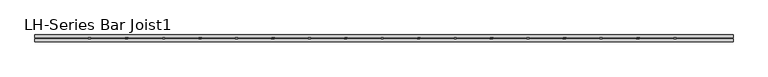
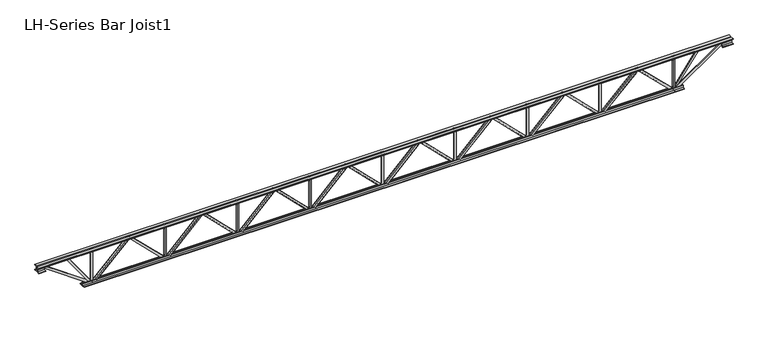
"""IFC4 building model written with IfcOpenShell, lengths in millimetres: beam geometry, LH-Series Bar Joist1 : 32LH-SP8."""

from ifc_helpers import new_model, si_unit, frame, origin, place, context, project, spatial, polyline, outline, extrude, faceted_brep, source, transform, mapped, element, save


def lh_series_bar_joist1_18190fb8(model_context):
    return source(origin(), model_context, "Body", "SolidModel", [
        extrude(outline(polyline([(406.4, 3276.6), (406.4, 3225.8), (323.85, 3225.8), (312.7375, 3236.9125), (-312.7375, 3236.9125), (-323.85, 3225.8), (-406.4, 3225.8), (-406.4, 3276.6), (406.4, 3276.6)])), frame((0.0, -12.7, 0.0), z_axis=(0.0, 1.0, 0.0), x_axis=(0.0, 0.0, 1.0)), (0.0, 0.0, 1.0), 25.4),
        faceted_brep([(3251.2, 0.0, -355.6), (3251.2, 0.0, -406.4), (3251.2, 12.7, -406.4), (3251.2, 12.7, -355.6), (3236.3210245, 0.0, -355.6), (2474.3210245, 0.0, 406.4), (2413.0, 0.0, 406.4), (2413.0, 0.0, 355.6), (2453.2789755, 0.0, 355.6), (3215.2789755, 0.0, -406.4), (3215.2789755, 12.7, -406.4), (3151.7789755, 12.7, -342.9), (3160.7592316, 12.7, -333.9197439), (2474.9592316, 12.7, 351.8802561), (2465.9789755, 12.7, 342.9), (2453.2789755, 12.7, 355.6), (2413.0, 12.7, 355.6), (2413.0, 12.7, 406.4), (2474.3210245, 12.7, 406.4), (3236.3210245, 12.7, -355.6), (2465.9789755, 50.8, 342.9), (3151.7789755, 50.8, -342.9), (3160.7592316, 50.8, -333.9197439), (2474.9592316, 50.8, 351.8802561)], [[[0, 1, 2, 3]], [[1, 0, 4, 5, 6, 7, 8, 9]], [[2, 1, 9, 10]], [[3, 2, 10, 11, 12, 13, 14, 15, 16, 17, 18, 19]], [[0, 3, 19, 4]], [[9, 8, 15, 14, 20, 21, 11, 10]], [[5, 4, 19, 18]], [[7, 6, 17, 16]], [[8, 7, 16, 15]], [[6, 5, 18, 17]], [[11, 21, 22, 12]], [[13, 23, 20, 14]], [[22, 21, 20, 23]], [[12, 22, 23, 13]]]),
        faceted_brep([(1625.6, -12.7, -355.6), (1625.6, 0.0, -355.6), (1625.6, 0.0, -406.4), (1625.6, -12.7, -406.4), (1640.4789755, -12.7, -355.6), (1640.4789755, 0.0, -355.6), (2402.4789755, 0.0, 406.4), (2463.8, 0.0, 406.4), (2463.8, 0.0, 355.6), (2423.5210245, 0.0, 355.6), (1661.5210245, 0.0, -406.4), (1661.5210245, -12.7, -406.4), (1725.0210245, -12.7, -342.9), (1716.0407684, -12.7, -333.9197439), (2401.8407684, -12.7, 351.8802561), (2410.8210245, -12.7, 342.9), (2423.5210245, -12.7, 355.6), (2463.8, -12.7, 355.6), (2463.8, -12.7, 406.4), (2402.4789755, -12.7, 406.4), (2410.8210245, -50.8, 342.9), (1725.0210245, -50.8, -342.9), (1716.0407684, -50.8, -333.9197439), (2401.8407684, -50.8, 351.8802561)], [[[0, 1, 2, 3]], [[1, 0, 4, 5]], [[2, 1, 5, 6, 7, 8, 9, 10]], [[3, 2, 10, 11]], [[0, 3, 11, 12, 13, 14, 15, 16, 17, 18, 19, 4]], [[5, 4, 19, 6]], [[10, 9, 16, 15, 20, 21, 12, 11]], [[8, 7, 18, 17]], [[7, 6, 19, 18]], [[9, 8, 17, 16]], [[21, 22, 13, 12]], [[20, 15, 14, 23]], [[22, 21, 20, 23]], [[13, 22, 23, 14]]]),
        extrude(outline(polyline([(406.4, 1651.0), (406.4, 1600.2), (323.85, 1600.2), (312.7375, 1611.3125), (-312.7375, 1611.3125), (-323.85, 1600.2), (-406.4, 1600.2), (-406.4, 1651.0), (406.4, 1651.0)])), frame((0.0, -12.7, 0.0), z_axis=(0.0, 1.0, 0.0), x_axis=(0.0, 0.0, 1.0)), (0.0, 0.0, 1.0), 25.4),
        faceted_brep([(1625.6, 0.0, -355.6), (1625.6, 0.0, -406.4), (1625.6, 12.7, -406.4), (1625.6, 12.7, -355.6), (1610.7210245, 0.0, -355.6), (848.7210245, 0.0, 406.4), (787.4, 0.0, 406.4), (787.4, 0.0, 355.6), (827.6789755, 0.0, 355.6), (1589.6789755, 0.0, -406.4), (1589.6789755, 12.7, -406.4), (1526.1789755, 12.7, -342.9), (1535.1592316, 12.7, -333.9197439), (849.3592316, 12.7, 351.8802561), (840.3789755, 12.7, 342.9), (827.6789755, 12.7, 355.6), (787.4, 12.7, 355.6), (787.4, 12.7, 406.4), (848.7210245, 12.7, 406.4), (1610.7210245, 12.7, -355.6), (840.3789755, 50.8, 342.9), (1526.1789755, 50.8, -342.9), (1535.1592316, 50.8, -333.9197439), (849.3592316, 50.8, 351.8802561)], [[[0, 1, 2, 3]], [[1, 0, 4, 5, 6, 7, 8, 9]], [[2, 1, 9, 10]], [[3, 2, 10, 11, 12, 13, 14, 15, 16, 17, 18, 19]], [[0, 3, 19, 4]], [[9, 8, 15, 14, 20, 21, 11, 10]], [[5, 4, 19, 18]], [[7, 6, 17, 16]], [[8, 7, 16, 15]], [[6, 5, 18, 17]], [[11, 21, 22, 12]], [[13, 23, 20, 14]], [[22, 21, 20, 23]], [[12, 22, 23, 13]]]),
        faceted_brep([(0.0, -12.7, -355.6), (0.0, 0.0, -355.6), (0.0, 0.0, -406.4), (0.0, -12.7, -406.4), (14.8789755, -12.7, -355.6), (14.8789755, 0.0, -355.6), (776.8789755, 0.0, 406.4), (838.2, 0.0, 406.4), (838.2, 0.0, 355.6), (797.9210245, 0.0, 355.6), (35.9210245, 0.0, -406.4), (35.9210245, -12.7, -406.4), (99.4210245, -12.7, -342.9), (90.4407684, -12.7, -333.9197439), (776.2407684, -12.7, 351.8802561), (785.2210245, -12.7, 342.9), (797.9210245, -12.7, 355.6), (838.2, -12.7, 355.6), (838.2, -12.7, 406.4), (776.8789755, -12.7, 406.4), (785.2210245, -50.8, 342.9), (99.4210245, -50.8, -342.9), (90.4407684, -50.8, -333.9197439), (776.2407684, -50.8, 351.8802561)], [[[0, 1, 2, 3]], [[1, 0, 4, 5]], [[2, 1, 5, 6, 7, 8, 9, 10]], [[3, 2, 10, 11]], [[0, 3, 11, 12, 13, 14, 15, 16, 17, 18, 19, 4]], [[5, 4, 19, 6]], [[10, 9, 16, 15, 20, 21, 12, 11]], [[8, 7, 18, 17]], [[7, 6, 19, 18]], [[9, 8, 17, 16]], [[21, 22, 13, 12]], [[20, 15, 14, 23]], [[22, 21, 20, 23]], [[13, 22, 23, 14]]]),
        extrude(outline(polyline([(406.4, 25.4), (406.4, -25.4), (323.85, -25.4), (312.7375, -14.2875), (-312.7375, -14.2875), (-323.85, -25.4), (-406.4, -25.4), (-406.4, 25.4), (406.4, 25.4)])), frame((0.0, -12.7, 0.0), z_axis=(0.0, 1.0, 0.0), x_axis=(0.0, 0.0, 1.0)), (0.0, 0.0, 1.0), 25.4),
        faceted_brep([(0.0, 0.0, -355.6), (0.0, 0.0, -406.4), (0.0, 12.7, -406.4), (0.0, 12.7, -355.6), (-14.8789755, 0.0, -355.6), (-776.8789755, 0.0, 406.4), (-838.2, 0.0, 406.4), (-838.2, 0.0, 355.6), (-797.9210245, 0.0, 355.6), (-35.9210245, 0.0, -406.4), (-35.9210245, 12.7, -406.4), (-99.4210245, 12.7, -342.9), (-90.4407684, 12.7, -333.9197439), (-776.2407684, 12.7, 351.8802561), (-785.2210245, 12.7, 342.9), (-797.9210245, 12.7, 355.6), (-838.2, 12.7, 355.6), (-838.2, 12.7, 406.4), (-776.8789755, 12.7, 406.4), (-14.8789755, 12.7, -355.6), (-785.2210245, 50.8, 342.9), (-99.4210245, 50.8, -342.9), (-90.4407684, 50.8, -333.9197439), (-776.2407684, 50.8, 351.8802561)], [[[0, 1, 2, 3]], [[1, 0, 4, 5, 6, 7, 8, 9]], [[2, 1, 9, 10]], [[3, 2, 10, 11, 12, 13, 14, 15, 16, 17, 18, 19]], [[0, 3, 19, 4]], [[9, 8, 15, 14, 20, 21, 11, 10]], [[5, 4, 19, 18]], [[7, 6, 17, 16]], [[8, 7, 16, 15]], [[6, 5, 18, 17]], [[11, 21, 22, 12]], [[13, 23, 20, 14]], [[22, 21, 20, 23]], [[12, 22, 23, 13]]]),
        faceted_brep([(-1625.6, -12.7, -355.6), (-1625.6, 0.0, -355.6), (-1625.6, 0.0, -406.4), (-1625.6, -12.7, -406.4), (-1610.7210245, -12.7, -355.6), (-1610.7210245, 0.0, -355.6), (-848.7210245, 0.0, 406.4), (-787.4, 0.0, 406.4), (-787.4, 0.0, 355.6), (-827.6789755, 0.0, 355.6), (-1589.6789755, 0.0, -406.4), (-1589.6789755, -12.7, -406.4), (-1526.1789755, -12.7, -342.9), (-1535.1592316, -12.7, -333.9197439), (-849.3592316, -12.7, 351.8802561), (-840.3789755, -12.7, 342.9), (-827.6789755, -12.7, 355.6), (-787.4, -12.7, 355.6), (-787.4, -12.7, 406.4), (-848.7210245, -12.7, 406.4), (-840.3789755, -50.8, 342.9), (-1526.1789755, -50.8, -342.9), (-1535.1592316, -50.8, -333.9197439), (-849.3592316, -50.8, 351.8802561)], [[[0, 1, 2, 3]], [[1, 0, 4, 5]], [[2, 1, 5, 6, 7, 8, 9, 10]], [[3, 2, 10, 11]], [[0, 3, 11, 12, 13, 14, 15, 16, 17, 18, 19, 4]], [[5, 4, 19, 6]], [[10, 9, 16, 15, 20, 21, 12, 11]], [[8, 7, 18, 17]], [[7, 6, 19, 18]], [[9, 8, 17, 16]], [[21, 22, 13, 12]], [[20, 15, 14, 23]], [[22, 21, 20, 23]], [[13, 22, 23, 14]]]),
        extrude(outline(polyline([(406.4, 6556.375), (406.4, 6505.575), (323.85, 6505.575), (312.7375, 6516.6875), (-312.7375, 6516.6875), (-323.85, 6505.575), (-406.4, 6505.575), (-406.4, 6556.375), (406.4, 6556.375)])), frame((0.0, -12.7, 0.0), z_axis=(0.0, 1.0, 0.0), x_axis=(0.0, 0.0, 1.0)), (0.0, 0.0, 1.0), 25.4),
        faceted_brep([(6530.975, 0.0, -355.6), (6530.975, 0.0, -406.4), (6530.975, 12.7, -406.4), (6530.975, 12.7, -355.6), (6515.958098, 0.0, -355.6), (5739.670598, 0.0, 406.4), (5678.4875, 0.0, 406.4), (5678.4875, 0.0, 355.6), (5718.904402, 0.0, 355.6), (6495.191902, 0.0, -406.4), (6495.191902, 12.7, -406.4), (6431.104883, 12.7, -343.4924966), (6440.0013474, 12.7, -334.4292234), (5740.6182703, 12.7, 352.0817725), (5731.7218059, 12.7, 343.0184993), (5718.904402, 12.7, 355.6), (5678.4875, 12.7, 355.6), (5678.4875, 12.7, 406.4), (5739.670598, 12.7, 406.4), (6515.958098, 12.7, -355.6), (5731.7218059, 50.8, 343.0184993), (6431.104883, 50.8, -343.4924966), (6440.0013474, 50.8, -334.4292234), (5740.6182703, 50.8, 352.0817725)], [[[0, 1, 2, 3]], [[1, 0, 4, 5, 6, 7, 8, 9]], [[2, 1, 9, 10]], [[3, 2, 10, 11, 12, 13, 14, 15, 16, 17, 18, 19]], [[0, 3, 19, 4]], [[9, 8, 15, 14, 20, 21, 11, 10]], [[5, 4, 19, 18]], [[7, 6, 17, 16]], [[8, 7, 16, 15]], [[6, 5, 18, 17]], [[11, 21, 22, 12]], [[13, 23, 20, 14]], [[22, 21, 20, 23]], [[12, 22, 23, 13]]]),
        faceted_brep([(4876.8, -12.7, -355.6), (4876.8, 0.0, -355.6), (4876.8, 0.0, -406.4), (4876.8, -12.7, -406.4), (4891.816902, -12.7, -355.6), (4891.816902, 0.0, -355.6), (5668.104402, 0.0, 406.4), (5729.2875, 0.0, 406.4), (5729.2875, 0.0, 355.6), (5688.870598, 0.0, 355.6), (4912.583098, 0.0, -406.4), (4912.583098, -12.7, -406.4), (4976.670117, -12.7, -343.4924966), (4967.7736526, -12.7, -334.4292234), (5667.1567297, -12.7, 352.0817725), (5676.0531941, -12.7, 343.0184993), (5688.870598, -12.7, 355.6), (5729.2875, -12.7, 355.6), (5729.2875, -12.7, 406.4), (5668.104402, -12.7, 406.4), (5676.0531941, -50.8, 343.0184993), (4976.670117, -50.8, -343.4924966), (4967.7736526, -50.8, -334.4292234), (5667.1567297, -50.8, 352.0817725)], [[[0, 1, 2, 3]], [[1, 0, 4, 5]], [[2, 1, 5, 6, 7, 8, 9, 10]], [[3, 2, 10, 11]], [[0, 3, 11, 12, 13, 14, 15, 16, 17, 18, 19, 4]], [[5, 4, 19, 6]], [[10, 9, 16, 15, 20, 21, 12, 11]], [[8, 7, 18, 17]], [[7, 6, 19, 18]], [[9, 8, 17, 16]], [[21, 22, 13, 12]], [[20, 15, 14, 23]], [[22, 21, 20, 23]], [[13, 22, 23, 14]]]),
        extrude(outline(polyline([(406.4, -4851.4), (406.4, -4902.2), (323.85, -4902.2), (312.7375, -4891.0875), (-312.7375, -4891.0875), (-323.85, -4902.2), (-406.4, -4902.2), (-406.4, -4851.4), (406.4, -4851.4)])), frame((0.0, -12.7, 0.0), z_axis=(0.0, 1.0, 0.0), x_axis=(0.0, 0.0, 1.0)), (0.0, 0.0, 1.0), 25.4),
        extrude(outline(polyline([(406.4, -6505.575), (406.4, -6556.375), (323.85, -6556.375), (312.7375, -6545.2625), (-312.7375, -6545.2625), (-323.85, -6556.375), (-406.4, -6556.375), (-406.4, -6505.575), (406.4, -6505.575)])), frame((0.0, -12.7, 0.0), z_axis=(0.0, 1.0, 0.0), x_axis=(0.0, 0.0, 1.0)), (0.0, 0.0, 1.0), 25.4),
        faceted_brep([(-4876.8, 0.0, -355.6), (-4876.8, 0.0, -406.4), (-4876.8, 12.7, -406.4), (-4876.8, 12.7, -355.6), (-4891.816902, 0.0, -355.6), (-5668.104402, 0.0, 406.4), (-5729.2875, 0.0, 406.4), (-5729.2875, 0.0, 355.6), (-5688.870598, 0.0, 355.6), (-4912.583098, 0.0, -406.4), (-4912.583098, 12.7, -406.4), (-4976.670117, 12.7, -343.4924966), (-4967.7736526, 12.7, -334.4292234), (-5667.1567297, 12.7, 352.0817725), (-5676.0531941, 12.7, 343.0184993), (-5688.870598, 12.7, 355.6), (-5729.2875, 12.7, 355.6), (-5729.2875, 12.7, 406.4), (-5668.104402, 12.7, 406.4), (-4891.816902, 12.7, -355.6), (-5676.0531941, 50.8, 343.0184993), (-4976.670117, 50.8, -343.4924966), (-4967.7736526, 50.8, -334.4292234), (-5667.1567297, 50.8, 352.0817725)], [[[0, 1, 2, 3]], [[1, 0, 4, 5, 6, 7, 8, 9]], [[2, 1, 9, 10]], [[3, 2, 10, 11, 12, 13, 14, 15, 16, 17, 18, 19]], [[0, 3, 19, 4]], [[9, 8, 15, 14, 20, 21, 11, 10]], [[5, 4, 19, 18]], [[7, 6, 17, 16]], [[8, 7, 16, 15]], [[6, 5, 18, 17]], [[11, 21, 22, 12]], [[13, 23, 20, 14]], [[22, 21, 20, 23]], [[12, 22, 23, 13]]]),
        faceted_brep([(-6530.975, -12.7, -355.6), (-6530.975, 0.0, -355.6), (-6530.975, 0.0, -406.4), (-6530.975, -12.7, -406.4), (-6515.958098, -12.7, -355.6), (-6515.958098, 0.0, -355.6), (-5739.670598, 0.0, 406.4), (-5678.4875, 0.0, 406.4), (-5678.4875, 0.0, 355.6), (-5718.904402, 0.0, 355.6), (-6495.191902, 0.0, -406.4), (-6495.191902, -12.7, -406.4), (-6431.104883, -12.7, -343.4924966), (-6440.0013474, -12.7, -334.4292234), (-5740.6182703, -12.7, 352.0817725), (-5731.7218059, -12.7, 343.0184993), (-5718.904402, -12.7, 355.6), (-5678.4875, -12.7, 355.6), (-5678.4875, -12.7, 406.4), (-5739.670598, -12.7, 406.4), (-5731.7218059, -50.8, 343.0184993), (-6431.104883, -50.8, -343.4924966), (-6440.0013474, -50.8, -334.4292234), (-5740.6182703, -50.8, 352.0817725)], [[[0, 1, 2, 3]], [[1, 0, 4, 5]], [[2, 1, 5, 6, 7, 8, 9, 10]], [[3, 2, 10, 11]], [[0, 3, 11, 12, 13, 14, 15, 16, 17, 18, 19, 4]], [[5, 4, 19, 6]], [[10, 9, 16, 15, 20, 21, 12, 11]], [[8, 7, 18, 17]], [[7, 6, 19, 18]], [[9, 8, 17, 16]], [[21, 22, 13, 12]], [[20, 15, 14, 23]], [[22, 21, 20, 23]], [[13, 22, 23, 14]]]),
        extrude(outline(polyline([(406.4, -1600.2), (406.4, -1651.0), (323.85, -1651.0), (312.7375, -1639.8875), (-312.7375, -1639.8875), (-323.85, -1651.0), (-406.4, -1651.0), (-406.4, -1600.2), (406.4, -1600.2)])), frame((0.0, -12.7, 0.0), z_axis=(0.0, 1.0, 0.0), x_axis=(0.0, 0.0, 1.0)), (0.0, 0.0, 1.0), 25.4),
        faceted_brep([(-1625.6, 0.0, -355.6), (-1625.6, 0.0, -406.4), (-1625.6, 12.7, -406.4), (-1625.6, 12.7, -355.6), (-1640.4789755, 0.0, -355.6), (-2402.4789755, 0.0, 406.4), (-2463.8, 0.0, 406.4), (-2463.8, 0.0, 355.6), (-2423.5210245, 0.0, 355.6), (-1661.5210245, 0.0, -406.4), (-1661.5210245, 12.7, -406.4), (-1725.0210245, 12.7, -342.9), (-1716.0407684, 12.7, -333.9197439), (-2401.8407684, 12.7, 351.8802561), (-2410.8210245, 12.7, 342.9), (-2423.5210245, 12.7, 355.6), (-2463.8, 12.7, 355.6), (-2463.8, 12.7, 406.4), (-2402.4789755, 12.7, 406.4), (-1640.4789755, 12.7, -355.6), (-2410.8210245, 50.8, 342.9), (-1725.0210245, 50.8, -342.9), (-1716.0407684, 50.8, -333.9197439), (-2401.8407684, 50.8, 351.8802561)], [[[0, 1, 2, 3]], [[1, 0, 4, 5, 6, 7, 8, 9]], [[2, 1, 9, 10]], [[3, 2, 10, 11, 12, 13, 14, 15, 16, 17, 18, 19]], [[0, 3, 19, 4]], [[9, 8, 15, 14, 20, 21, 11, 10]], [[5, 4, 19, 18]], [[7, 6, 17, 16]], [[8, 7, 16, 15]], [[6, 5, 18, 17]], [[11, 21, 22, 12]], [[13, 23, 20, 14]], [[22, 21, 20, 23]], [[12, 22, 23, 13]]]),
        faceted_brep([(-3251.2, -12.7, -355.6), (-3251.2, 0.0, -355.6), (-3251.2, 0.0, -406.4), (-3251.2, -12.7, -406.4), (-3236.3210245, -12.7, -355.6), (-3236.3210245, 0.0, -355.6), (-2474.3210245, 0.0, 406.4), (-2413.0, 0.0, 406.4), (-2413.0, 0.0, 355.6), (-2453.2789755, 0.0, 355.6), (-3215.2789755, 0.0, -406.4), (-3215.2789755, -12.7, -406.4), (-3151.7789755, -12.7, -342.9), (-3160.7592316, -12.7, -333.9197439), (-2474.9592316, -12.7, 351.8802561), (-2465.9789755, -12.7, 342.9), (-2453.2789755, -12.7, 355.6), (-2413.0, -12.7, 355.6), (-2413.0, -12.7, 406.4), (-2474.3210245, -12.7, 406.4), (-2465.9789755, -50.8, 342.9), (-3151.7789755, -50.8, -342.9), (-3160.7592316, -50.8, -333.9197439), (-2474.9592316, -50.8, 351.8802561)], [[[0, 1, 2, 3]], [[1, 0, 4, 5]], [[2, 1, 5, 6, 7, 8, 9, 10]], [[3, 2, 10, 11]], [[0, 3, 11, 12, 13, 14, 15, 16, 17, 18, 19, 4]], [[5, 4, 19, 6]], [[10, 9, 16, 15, 20, 21, 12, 11]], [[8, 7, 18, 17]], [[7, 6, 19, 18]], [[9, 8, 17, 16]], [[21, 22, 13, 12]], [[20, 15, 14, 23]], [[22, 21, 20, 23]], [[13, 22, 23, 14]]]),
        extrude(outline(polyline([(406.4, 4902.2), (406.4, 4851.4), (323.85, 4851.4), (312.7375, 4862.5125), (-312.7375, 4862.5125), (-323.85, 4851.4), (-406.4, 4851.4), (-406.4, 4902.2), (406.4, 4902.2)])), frame((0.0, -12.7, 0.0), z_axis=(0.0, 1.0, 0.0), x_axis=(0.0, 0.0, 1.0)), (0.0, 0.0, 1.0), 25.4),
        faceted_brep([(4876.8, 0.0, -355.6), (4876.8, 0.0, -406.4), (4876.8, 12.7, -406.4), (4876.8, 12.7, -355.6), (4861.9210245, 0.0, -355.6), (4099.9210245, 0.0, 406.4), (4038.6, 0.0, 406.4), (4038.6, 0.0, 355.6), (4078.8789755, 0.0, 355.6), (4840.8789755, 0.0, -406.4), (4840.8789755, 12.7, -406.4), (4777.3789755, 12.7, -342.9), (4786.3592316, 12.7, -333.9197439), (4100.5592316, 12.7, 351.8802561), (4091.5789755, 12.7, 342.9), (4078.8789755, 12.7, 355.6), (4038.6, 12.7, 355.6), (4038.6, 12.7, 406.4), (4099.9210245, 12.7, 406.4), (4861.9210245, 12.7, -355.6), (4091.5789755, 50.8, 342.9), (4777.3789755, 50.8, -342.9), (4786.3592316, 50.8, -333.9197439), (4100.5592316, 50.8, 351.8802561)], [[[0, 1, 2, 3]], [[1, 0, 4, 5, 6, 7, 8, 9]], [[2, 1, 9, 10]], [[3, 2, 10, 11, 12, 13, 14, 15, 16, 17, 18, 19]], [[0, 3, 19, 4]], [[9, 8, 15, 14, 20, 21, 11, 10]], [[5, 4, 19, 18]], [[7, 6, 17, 16]], [[8, 7, 16, 15]], [[6, 5, 18, 17]], [[11, 21, 22, 12]], [[13, 23, 20, 14]], [[22, 21, 20, 23]], [[12, 22, 23, 13]]]),
        faceted_brep([(3251.2, -12.7, -355.6), (3251.2, 0.0, -355.6), (3251.2, 0.0, -406.4), (3251.2, -12.7, -406.4), (3266.0789755, -12.7, -355.6), (3266.0789755, 0.0, -355.6), (4028.0789755, 0.0, 406.4), (4089.4, 0.0, 406.4), (4089.4, 0.0, 355.6), (4049.1210245, 0.0, 355.6), (3287.1210245, 0.0, -406.4), (3287.1210245, -12.7, -406.4), (3350.6210245, -12.7, -342.9), (3341.6407684, -12.7, -333.9197439), (4027.4407684, -12.7, 351.8802561), (4036.4210245, -12.7, 342.9), (4049.1210245, -12.7, 355.6), (4089.4, -12.7, 355.6), (4089.4, -12.7, 406.4), (4028.0789755, -12.7, 406.4), (4036.4210245, -50.8, 342.9), (3350.6210245, -50.8, -342.9), (3341.6407684, -50.8, -333.9197439), (4027.4407684, -50.8, 351.8802561)], [[[0, 1, 2, 3]], [[1, 0, 4, 5]], [[2, 1, 5, 6, 7, 8, 9, 10]], [[3, 2, 10, 11]], [[0, 3, 11, 12, 13, 14, 15, 16, 17, 18, 19, 4]], [[5, 4, 19, 6]], [[10, 9, 16, 15, 20, 21, 12, 11]], [[8, 7, 18, 17]], [[7, 6, 19, 18]], [[9, 8, 17, 16]], [[21, 22, 13, 12]], [[20, 15, 14, 23]], [[22, 21, 20, 23]], [[13, 22, 23, 14]]]),
        extrude(outline(polyline([(406.4, -3225.8), (406.4, -3276.6), (323.85, -3276.6), (312.7375, -3265.4875), (-312.7375, -3265.4875), (-323.85, -3276.6), (-406.4, -3276.6), (-406.4, -3225.8), (406.4, -3225.8)])), frame((0.0, -12.7, 0.0), z_axis=(0.0, 1.0, 0.0), x_axis=(0.0, 0.0, 1.0)), (0.0, 0.0, 1.0), 25.4),
        faceted_brep([(-3251.2, 0.0, -355.6), (-3251.2, 0.0, -406.4), (-3251.2, 12.7, -406.4), (-3251.2, 12.7, -355.6), (-3266.0789755, 0.0, -355.6), (-4028.0789755, 0.0, 406.4), (-4089.4, 0.0, 406.4), (-4089.4, 0.0, 355.6), (-4049.1210245, 0.0, 355.6), (-3287.1210245, 0.0, -406.4), (-3287.1210245, 12.7, -406.4), (-3350.6210245, 12.7, -342.9), (-3341.6407684, 12.7, -333.9197439), (-4027.4407684, 12.7, 351.8802561), (-4036.4210245, 12.7, 342.9), (-4049.1210245, 12.7, 355.6), (-4089.4, 12.7, 355.6), (-4089.4, 12.7, 406.4), (-4028.0789755, 12.7, 406.4), (-3266.0789755, 12.7, -355.6), (-4036.4210245, 50.8, 342.9), (-3350.6210245, 50.8, -342.9), (-3341.6407684, 50.8, -333.9197439), (-4027.4407684, 50.8, 351.8802561)], [[[0, 1, 2, 3]], [[1, 0, 4, 5, 6, 7, 8, 9]], [[2, 1, 9, 10]], [[3, 2, 10, 11, 12, 13, 14, 15, 16, 17, 18, 19]], [[0, 3, 19, 4]], [[9, 8, 15, 14, 20, 21, 11, 10]], [[5, 4, 19, 18]], [[7, 6, 17, 16]], [[8, 7, 16, 15]], [[6, 5, 18, 17]], [[11, 21, 22, 12]], [[13, 23, 20, 14]], [[22, 21, 20, 23]], [[12, 22, 23, 13]]]),
        faceted_brep([(-4876.8, -12.7, -355.6), (-4876.8, 0.0, -355.6), (-4876.8, 0.0, -406.4), (-4876.8, -12.7, -406.4), (-4861.9210245, -12.7, -355.6), (-4861.9210245, 0.0, -355.6), (-4099.9210245, 0.0, 406.4), (-4038.6, 0.0, 406.4), (-4038.6, 0.0, 355.6), (-4078.8789755, 0.0, 355.6), (-4840.8789755, 0.0, -406.4), (-4840.8789755, -12.7, -406.4), (-4777.3789755, -12.7, -342.9), (-4786.3592316, -12.7, -333.9197439), (-4100.5592316, -12.7, 351.8802561), (-4091.5789755, -12.7, 342.9), (-4078.8789755, -12.7, 355.6), (-4038.6, -12.7, 355.6), (-4038.6, -12.7, 406.4), (-4099.9210245, -12.7, 406.4), (-4091.5789755, -50.8, 342.9), (-4777.3789755, -50.8, -342.9), (-4786.3592316, -50.8, -333.9197439), (-4100.5592316, -50.8, 351.8802561)], [[[0, 1, 2, 3]], [[1, 0, 4, 5]], [[2, 1, 5, 6, 7, 8, 9, 10]], [[3, 2, 10, 11]], [[0, 3, 11, 12, 13, 14, 15, 16, 17, 18, 19, 4]], [[5, 4, 19, 6]], [[10, 9, 16, 15, 20, 21, 12, 11]], [[8, 7, 18, 17]], [[7, 6, 19, 18]], [[9, 8, 17, 16]], [[21, 22, 13, 12]], [[20, 15, 14, 23]], [[22, 21, 20, 23]], [[13, 22, 23, 14]]]),
        extrude(outline(polyline([(12.7, 406.4), (76.2, 406.4), (76.2, 393.7), (25.4, 393.7), (25.4, 342.9), (12.7, 342.9), (12.7, 406.4)])), frame((-7750.175, 0.0, 0.0), z_axis=(1.0, 0.0, 0.0), x_axis=(0.0, 1.0, 0.0)), (0.0, 0.0, 1.0), 15576.55),
        extrude(outline(polyline([(-12.7, 406.4), (-12.7, 342.9), (-25.4, 342.9), (-25.4, 393.7), (-76.2, 393.7), (-76.2, 406.4), (-12.7, 406.4)])), frame((-7750.175, 0.0, 0.0), z_axis=(1.0, 0.0, 0.0), x_axis=(0.0, 1.0, 0.0)), (0.0, 0.0, 1.0), 15576.55),
        extrude(outline(polyline([(-12.7, 279.4), (-76.2, 279.4), (-76.2, 292.1), (-25.4, 292.1), (-25.4, 342.9), (-12.7, 342.9), (-12.7, 279.4)])), frame((-7750.175, 0.0, 0.0), z_axis=(1.0, 0.0, 0.0), x_axis=(0.0, 1.0, 0.0)), (0.0, 0.0, 1.0), 152.4),
        extrude(outline(polyline([(76.2, 279.4), (12.7, 279.4), (12.7, 342.9), (25.4, 342.9), (25.4, 292.1), (76.2, 292.1), (76.2, 279.4)])), frame((-7750.175, 0.0, 0.0), z_axis=(1.0, 0.0, 0.0), x_axis=(0.0, 1.0, 0.0)), (0.0, 0.0, 1.0), 152.4),
        extrude(outline(polyline([(12.7, 279.4), (12.7, 342.9), (25.4, 342.9), (25.4, 292.1), (76.2, 292.1), (76.2, 279.4), (12.7, 279.4)])), frame((7597.775, 0.0, 0.0), z_axis=(1.0, 0.0, 0.0), x_axis=(0.0, 1.0, 0.0)), (0.0, 0.0, 1.0), 228.6),
        extrude(outline(polyline([(-12.7, 279.4), (-76.2, 279.4), (-76.2, 292.1), (-25.4, 292.1), (-25.4, 342.9), (-12.7, 342.9), (-12.7, 279.4)])), frame((7597.775, 0.0, 0.0), z_axis=(1.0, 0.0, 0.0), x_axis=(0.0, 1.0, 0.0)), (0.0, 0.0, 1.0), 228.6),
        extrude(outline(polyline([(12.7, -406.4), (12.7, -342.9), (25.4, -342.9), (25.4, -393.7), (76.2, -393.7), (76.2, -406.4), (12.7, -406.4)])), frame((-6734.175, 0.0, 0.0), z_axis=(1.0, 0.0, 0.0), x_axis=(0.0, 1.0, 0.0)), (0.0, 0.0, 1.0), 13468.35),
        extrude(outline(polyline([(-12.7, -406.4), (-76.2, -406.4), (-76.2, -393.7), (-25.4, -393.7), (-25.4, -342.9), (-12.7, -342.9), (-12.7, -406.4)])), frame((-6734.175, 0.0, 0.0), z_axis=(1.0, 0.0, 0.0), x_axis=(0.0, 1.0, 0.0)), (0.0, 0.0, 1.0), 13468.35),
        extrude(outline(polyline([(6.35, -25.4), (-6.35, -25.4), (-6.35, 25.4), (6.35, 25.4), (6.35, -25.4)])), frame((-6530.975, 0.0, -400.05), z_axis=(-0.58320678309139, 0.0, 0.8123237335915974), x_axis=(0.0, -1.0, 0.0)), (0.0, 0.0, 1.0), 914.598416),
        extrude(outline(polyline([(0.0, -12.7), (0.0, 0.0), (1300.0142086, 0.0), (1300.0142086, -12.7), (0.0, -12.7)])), frame((-7612.2909413, 6.35, 322.056597), z_axis=(0.5714937537595753, 0.0, 0.8206064156547828), x_axis=(0.8206064156547828, 0.0, -0.5714937537595753)), (0.0, 0.0, 1.0), 50.8),
        extrude(outline(polyline([(6.35, 25.4), (6.35, -25.4), (-6.35, -25.4), (-6.35, 25.4), (6.35, 25.4)])), frame((6530.975, 0.0, -400.05), z_axis=(0.5811065900870399, 0.0, 0.8138274577313137), x_axis=(0.0, -1.0, 0.0)), (0.0, 0.0, 1.0), 912.9084955),
        extrude(outline(polyline([(0.0, -12.7), (0.0, 0.0), (1300.0142086, 0.0), (1300.0142086, -12.7), (0.0, -12.7)])), frame((6545.4909413, -6.35, -420.893403), z_axis=(-0.5714937537593278, 0.0, 0.8206064156549552), x_axis=(0.8206064156549552, 0.0, 0.5714937537593278)), (0.0, 0.0, 1.0), 50.8),
    ])


if __name__ == "__main__":
    model = new_model("IFC4")
    model_context = context("Model", 3, world=origin())
    ifc_project = project(units=[si_unit("LENGTHUNIT", "METRE", prefix="MILLI")], contexts=[model_context])
    site = spatial("IfcSite", under=ifc_project)
    building = spatial("IfcBuilding", under=site)
    placement = place(None, origin())
    lh_series_bar_joist1_shape = lh_series_bar_joist1_18190fb8(model_context)
    element("IfcBeam", 1, ObjectType="LH-Series Bar Joist1 : 32LH-SP8", at=placement, inside=building, context=model_context, shape_type="MappedRepresentation", body=[
        mapped(lh_series_bar_joist1_shape, transform((0.0, 0.0, 0.0), x_axis=(1.0, 0.0, 0.0), y_axis=(0.0, 1.0, 0.0), z_axis=(0.0, 0.0, 1.0))),
    ])
    save(model, "model.ifc")

# Revit data of these elements
# Type "LH-Series Bar Joist1 : 32LH-SP8"
#   Assembly Code = "B1010350"
#   Wt = 21
#   Web Thickness = 0' - 1"
#   Variable Panel [instance default] = 5' - 4"
#   Start Offset [instance default] = 0' - 0"
#   Start Extension [instance default] = 0' - 0"
#   Seat Length = 0' - 6"
#   Seat Depth = 0' - 5"
#   IntPanelWidth [instance default] = 5' - 4"
#   IntPanelArrayLength [instance default] = 21' - 4"
#   PanelAreaLength [instance default] = 32' - 0"
#   End Panel = 4' - 0"
#   End Offset [instance default] = 0' - 0"
#   End Extension [instance default] = 0' - 0"
#   Cord Leg = 0' - 2 1/2"
#   Chord Thickness = 0' - 0 1/2"
#   Length [instance default] = 40' - 0"
#   Depth = 2' - 8"
#   Vertical Member Visibility = yes
#   IntPanelArrayNum [instance default] = 4
#   Structural Material = none
# Element 1 (IfcBeam, "LH-Series Bar Joist1 : 32LH-SP8")
#   Variable Panel = 5' - 5 1/8"
#   IntPanelArrayLength = 32' - 0"
#   PanelAreaLength = 42' - 10 1/4"
#   End Extension = 0' - 3"
#   Length = 50' - 10 1/4"
#   IntPanelArrayNum = 6
